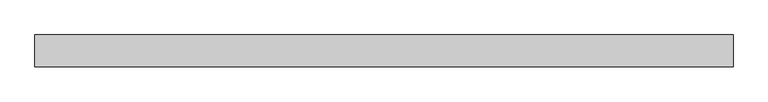
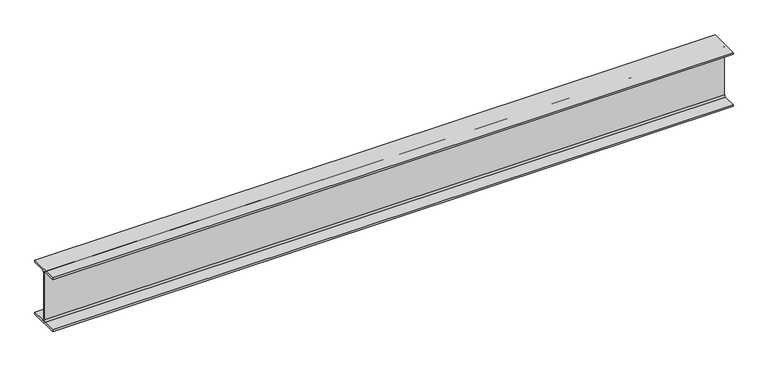
"""IFC4 building model written with IfcOpenShell, lengths in millimetres: beam geometry, Old_Steel Beam_H-KSD3502 : H_SB_ASB_H-200×200x8x12."""

import ifcopenshell
import ifcopenshell.guid

model = None  # the IFC model being written
_history = None  # IfcOwnerHistory: only IFC2X3 demands one
_inside = {}  # id of a spatial element -> (the spatial element, [elements in it])
_under = {}  # id of a project, library or spatial element -> (it, [spatial elements below it])
_declared = {}  # id of a project -> (the project, [libraries it declares])
_typed = {}  # id of a type object -> (the type object, [elements of that type])
_made_of = {}  # id of a material, layer set ... -> (it, [elements and type objects made of it])


def new_model(schema):
    """Start an empty IFC model of exactly this schema.

    Asked for "IFC4X3", IfcOpenShell would pick the latest addendum, in which some entities
    have other attributes; the version numbers below select the first issue.
    IFC2X3 requires an IfcOwnerHistory on every rooted entity: one is made here for all.
    """
    global model, _history
    if schema == "IFC4X3":
        model = ifcopenshell.file(schema_version=(4, 3, 0, 0))
    else:
        model = ifcopenshell.file(schema=schema)
    _inside.clear()
    _under.clear()
    _declared.clear()
    _typed.clear()
    _made_of.clear()
    _history = None
    if model.schema == "IFC2X3":
        org = make("IfcOrganization", Name="unknown")
        user = make(
            "IfcPersonAndOrganization",
            ThePerson=make("IfcPerson", FamilyName="unknown"),
            TheOrganization=org,
        )
        app = make(
            "IfcApplication",
            ApplicationDeveloper=org,
            Version="unknown",
            ApplicationFullName="unknown",
            ApplicationIdentifier="unknown",
        )
        _history = make(
            "IfcOwnerHistory",
            OwningUser=user,
            OwningApplication=app,
            ChangeAction="ADDED",
            CreationDate=0,
        )
    return model


def make(cls, **values):
    """One entity of the class cls with the attributes given. An attribute that is None is left unset."""
    return model.create_entity(
        cls, **{name: value for name, value in values.items() if value is not None}
    )


def rooted(cls, **values):
    """An entity with a GlobalId (a new one), such as an element, a storey or a relation."""
    return make(cls, GlobalId=ifcopenshell.guid.new(), OwnerHistory=_history, **values)


def si_unit(unit_type, name, prefix=None):
    """IfcSIUnit, for example si_unit("LENGTHUNIT", "METRE", prefix="MILLI")."""
    return make("IfcSIUnit", UnitType=unit_type, Prefix=prefix, Name=name)


def assignment(units):
    """IfcUnitAssignment: the units of a project."""
    return None if units is None else make("IfcUnitAssignment", Units=units)


def point(xyz):
    """IfcCartesianPoint."""
    return None if xyz is None else make("IfcCartesianPoint", Coordinates=xyz)


def direction(xyz):
    """IfcDirection."""
    return None if xyz is None else make("IfcDirection", DirectionRatios=xyz)


def frame(location, z_axis=None, x_axis=None):
    """IfcAxis2Placement3D, a coordinate frame: its origin and axes. An axis left out is left unset."""
    return make(
        "IfcAxis2Placement3D",
        Location=point(location),
        Axis=direction(z_axis),
        RefDirection=direction(x_axis),
    )


def frame_2d(location, x_axis=None):
    """IfcAxis2Placement2D, a coordinate frame in the plane: its origin and x axis."""
    return make(
        "IfcAxis2Placement2D", Location=point(location), RefDirection=direction(x_axis)
    )


def origin():
    """The frame at (0, 0, 0) with its axes left unset."""
    return frame((0.0, 0.0, 0.0))


def place(relative_to, where):
    """IfcLocalPlacement: puts the frame where relative to a parent placement (None: the world)."""
    return make(
        "IfcLocalPlacement", PlacementRelTo=relative_to, RelativePlacement=where
    )


def context(
    kind, dimensions, precision=None, world=None, true_north=None, identifier=None
):
    """IfcGeometricRepresentationContext, for example the 3D "Model" context."""
    return make(
        "IfcGeometricRepresentationContext",
        ContextIdentifier=identifier,
        ContextType=kind,
        CoordinateSpaceDimension=dimensions,
        Precision=precision,
        WorldCoordinateSystem=world,
        TrueNorth=true_north,
    )


def project(units=None, contexts=None):
    """IfcProject with its units and contexts."""
    return rooted(
        "IfcProject",
        Name="project",
        RepresentationContexts=contexts,
        UnitsInContext=assignment(units),
    )


def spatial(cls, under=None, at=None, **own):
    """A site, building, storey or space (cls), placed at a placement, below another one or the project."""
    s = rooted(cls, ObjectPlacement=at, **own)
    if under is not None:
        _under.setdefault(under.id(), (under, []))[1].append(s)
    return s


def polyline(points):
    """IfcPolyline through the points."""
    return make("IfcPolyline", Points=[point(p) for p in points])


def circle_curve(where, radius):
    """IfcCircle in the frame where."""
    return make("IfcCircle", Position=where, Radius=radius)


def trimmed(basis, trim1, trim2, sense, master):
    """IfcTrimmedCurve: the piece of a basis curve between two trims."""
    return make(
        "IfcTrimmedCurve",
        BasisCurve=basis,
        Trim1=trim1,
        Trim2=trim2,
        SenseAgreement=sense,
        MasterRepresentation=master,
    )


def segment(curve, same_sense, transition):
    """IfcCompositeCurveSegment."""
    return make(
        "IfcCompositeCurveSegment",
        Transition=transition,
        SameSense=same_sense,
        ParentCurve=curve,
    )


def composite_curve(segments, self_intersect=None):
    """IfcCompositeCurve: segments joined end to end."""
    return make("IfcCompositeCurve", Segments=segments, SelfIntersect=self_intersect)


def outline(outer, holes=None, kind="AREA"):
    """IfcArbitraryClosedProfileDef: a profile drawn as a closed curve; with holes, ...WithVoids."""
    if holes is None:
        return make("IfcArbitraryClosedProfileDef", ProfileType=kind, OuterCurve=outer)
    return make(
        "IfcArbitraryProfileDefWithVoids",
        ProfileType=kind,
        OuterCurve=outer,
        InnerCurves=holes,
    )


def extrude(swept, where, along, depth):
    """IfcExtrudedAreaSolid: the profile swept, set in the frame where, extruded along a direction by depth."""
    return make(
        "IfcExtrudedAreaSolid",
        SweptArea=swept,
        Position=where,
        ExtrudedDirection=direction(along),
        Depth=depth,
    )


def shape(context_of_items, identifier, shape_type, items):
    """IfcShapeRepresentation: the items that make up one representation, for example the "Body"."""
    return make(
        "IfcShapeRepresentation",
        ContextOfItems=context_of_items,
        RepresentationIdentifier=identifier,
        RepresentationType=shape_type,
        Items=items,
    )


def source(mapping_origin, context_of_items, identifier, shape_type, items):
    """IfcRepresentationMap: a shape defined once, which mapped items show again and again."""
    return make(
        "IfcRepresentationMap",
        MappingOrigin=mapping_origin,
        MappedRepresentation=shape(context_of_items, identifier, shape_type, items),
    )


def transform(
    local_origin,
    x_axis=None,
    y_axis=None,
    z_axis=None,
    scale=None,
    scale2=None,
    scale3=None,
    uniform=True,
):
    """IfcCartesianTransformationOperator3D, or its non-uniform kind. x_axis, y_axis, z_axis: its Axis1, 2, 3."""
    if uniform:
        return make(
            "IfcCartesianTransformationOperator3D",
            Axis1=direction(x_axis),
            Axis2=direction(y_axis),
            LocalOrigin=point(local_origin),
            Scale=scale,
            Axis3=direction(z_axis),
        )
    return make(
        "IfcCartesianTransformationOperator3DnonUniform",
        Axis1=direction(x_axis),
        Axis2=direction(y_axis),
        LocalOrigin=point(local_origin),
        Scale=scale,
        Axis3=direction(z_axis),
        Scale2=scale2,
        Scale3=scale3,
    )


def mapped(mapping_source, mapping_target):
    """IfcMappedItem: shows the shape of a source again, moved by a transform."""
    return make(
        "IfcMappedItem", MappingSource=mapping_source, MappingTarget=mapping_target
    )


def made_of(thing, what):
    """Note that an element or type object is made of a material, layer set ...; save() writes the relation."""
    if what is not None:
        _made_of.setdefault(what.id(), (what, []))[1].append(thing)
    return thing


def element(
    cls,
    number,
    at=None,
    inside=None,
    cuts=None,
    type_object=None,
    material=None,
    context=None,
    identifier="Body",
    shape_type=None,
    held_by="IfcProductDefinitionShape",
    body=None,
    shapes=None,
    **own,
):
    """One element of the class cls, such as IfcWall. Its Tag is "e" and its number.

    at: its placement. inside: the storey or other place that contains it. cuts: it is an
    opening in that element (IfcRelVoidsElement). A single representation is given by context,
    identifier, shape_type and body (its items); several are given by shapes. held_by: the class
    of the entity that holds the representations. save() writes the other relations.
    """
    e = rooted(cls, Tag="e%d" % number, ObjectPlacement=at, **own)
    if body is not None:
        shapes = [shape(context, identifier, shape_type, body)]
    if shapes is not None:
        e.Representation = make(held_by, Representations=shapes)
    if inside is not None:
        _inside.setdefault(inside.id(), (inside, []))[1].append(e)
    if cuts is not None:
        rooted(
            "IfcRelVoidsElement", RelatingBuildingElement=cuts, RelatedOpeningElement=e
        )
    if type_object is not None:
        _typed.setdefault(type_object.id(), (type_object, []))[1].append(e)
    return made_of(e, material)


def aggregate(whole, parts):
    """IfcRelAggregates: a whole, such as a stair, and the parts it consists of."""
    return rooted("IfcRelAggregates", RelatingObject=whole, RelatedObjects=parts)


def save(model, path):
    """Write the relations noted so far, then the file.

    IfcRelAggregates (storeys below a building ...), IfcRelContainedInSpatialStructure (elements
    in a storey), IfcRelDefinesByType, IfcRelAssociatesMaterial and IfcRelDeclares: one each for
    every whole, place, type object, material and project.
    """
    for whole, parts in _under.values():
        aggregate(whole, parts)
    for where, things in _inside.values():
        rooted(
            "IfcRelContainedInSpatialStructure",
            RelatedElements=things,
            RelatingStructure=where,
        )
    for kind, things in _typed.values():
        rooted("IfcRelDefinesByType", RelatedObjects=things, RelatingType=kind)
    for what, things in _made_of.values():
        rooted("IfcRelAssociatesMaterial", RelatedObjects=things, RelatingMaterial=what)
    for by, libraries in _declared.values():
        rooted("IfcRelDeclares", RelatingContext=by, RelatedDefinitions=libraries)
    model.write(path)


def beam_a769b179(model_context):
    return source(origin(), model_context, "Body", "SweptSolid", [
        extrude(outline(composite_curve([segment(polyline([(82.5, -141.5), (82.5, -151.7), (-82.5, -151.7), (-82.5, -141.5), (-11.9, -141.5)]), True, "CONTINUOUS"), segment(trimmed(circle_curve(frame_2d((-11.9, -132.6)), 8.9), [point((-11.9, -141.5))], [point((-3.0, -132.6))], True, "CARTESIAN"), True, "CONTINUOUS"), segment(polyline([(-3.0, -132.6), (-3.0, 132.6)]), True, "CONTINUOUS"), segment(trimmed(circle_curve(frame_2d((-11.9, 132.6)), 8.9), [point((-3.0, 132.6))], [point((-11.9, 141.5))], True, "CARTESIAN"), True, "CONTINUOUS"), segment(polyline([(-11.9, 141.5), (-82.5, 141.5), (-82.5, 151.7), (82.5, 151.7), (82.5, 141.5), (11.9, 141.5)]), True, "CONTINUOUS"), segment(trimmed(circle_curve(frame_2d((11.9, 132.6)), 8.9), [point((11.9, 141.5))], [point((3.0, 132.6))], True, "CARTESIAN"), True, "CONTINUOUS"), segment(polyline([(3.0, 132.6), (3.0, -132.6)]), True, "CONTINUOUS"), segment(trimmed(circle_curve(frame_2d((11.9, -132.6)), 8.9), [point((3.0, -132.6))], [point((11.9, -141.5))], True, "CARTESIAN"), True, "CONTINUOUS"), segment(polyline([(11.9, -141.5), (82.5, -141.5)]), True, "CONTINUOUS")], self_intersect=False)), frame((-1907.7947202, 0.0, 0.0), z_axis=(1.0, 0.0, 0.0), x_axis=(0.0, 1.0, 0.0)), (0.0, 0.0, 1.0), 3628.373533),
    ])


if __name__ == "__main__":
    model = new_model("IFC4")
    model_context = context("Model", 3, world=origin())
    ifc_project = project(units=[si_unit("LENGTHUNIT", "METRE", prefix="MILLI")], contexts=[model_context])
    site = spatial("IfcSite", under=ifc_project)
    building = spatial("IfcBuilding", under=site)
    placement = place(None, origin())
    beam_shape = beam_a769b179(model_context)
    element("IfcBeam", 1, ObjectType="Old_Steel Beam_H-KSD3502 : H_SB_ASB_H-200×200x8x12", at=placement, inside=building, context=model_context, shape_type="MappedRepresentation", body=[
        mapped(beam_shape, transform((0.0, 0.0, 0.0), x_axis=(1.0, 0.0, 0.0), y_axis=(0.0, 1.0, 0.0), z_axis=(0.0, 0.0, 1.0))),
    ])
    save(model, "model.ifc")

# Revit data of these elements
# Type "Old_Steel Beam_H-KSD3502 : H_SB_ASB_H-200×200x8x12"
#   Width = 20.0 cm
#   Web Thickness = 0.8 cm
#   Web Fillet = 1.3 cm
#   Warping Constant = 141376.0 cm⁶
#   Torsional Moment of Inertia = 26.2485 cm⁴
#   Torsional Modulus = 1.0 cm³
#   Section Area = 63.53 cm²
#   Plastic Modulus weak axis = 244.0 cm³
#   Plastic Modulus strong axis = 525.0 cm³
#   Perimeter = 1.16 m²/m
#   Nominal Weight = 49.90 kgf/m
#   Moment of Inertia weak axis = 1600.00 cm⁴
#   Moment of Inertia strong axis = 4720.00 cm⁴
#   Height = 20.0 cm
#   Flange Thickness = 1.2 cm
#   Elastic Modulus weak axis = 160.0 cm³
#   Elastic Modulus strong axis = 472.0 cm³
#   Centroid Vertical = 10.0 cm
#   Centroid Horizontal = 10.0 cm
#   Length [instance default] = 1.5240 m
#   Structural Material [instance default] = Steel, 45-345
#   Assembly Code = ""
# Element 1 (IfcBeam, "Old_Steel Beam_H-KSD3502 : H_SB_ASB_H-200×200x8x12")
#   Structural Material = none
# Materials
#   "Steel, 45-345": class "Metal", colour RGB 189 187 185, transparency 0, Description = "Steel 345 MPa", Cost = 0
